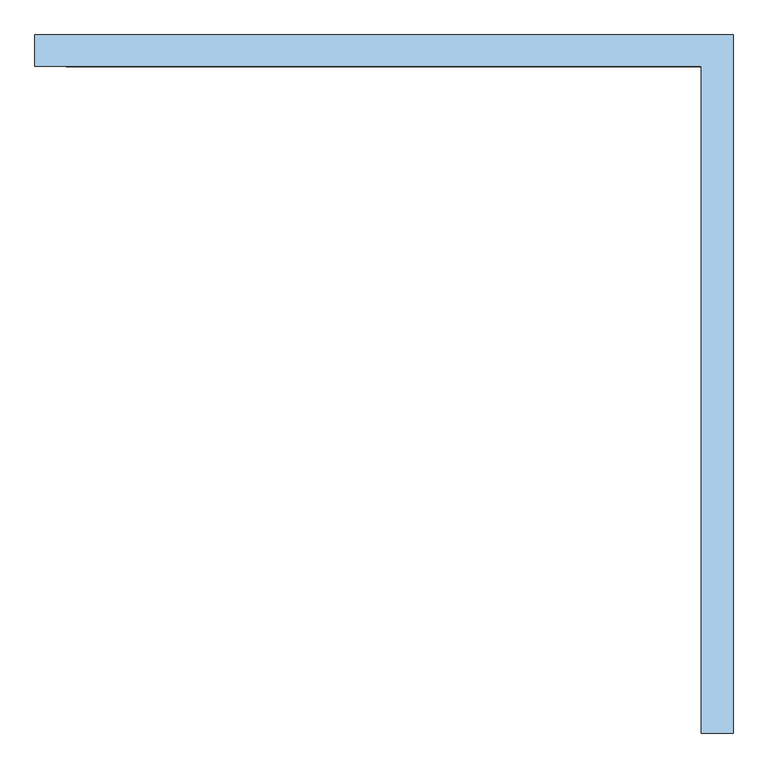
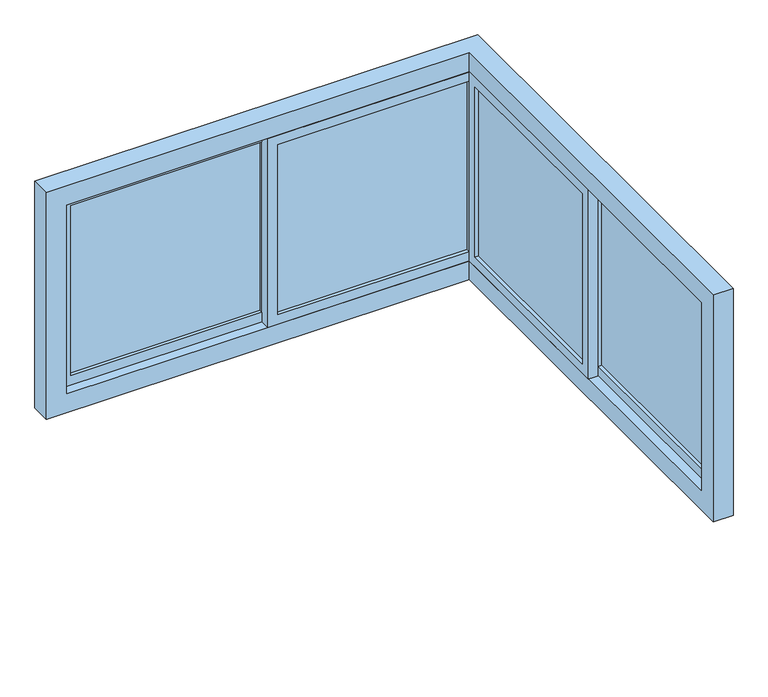
"""IFC4 building model written with IfcOpenShell, lengths in millimetres: window geometry, .CC_ND 300_JANELA DE CANTO_4 FOLHAS DE CORRER_VIDRO : 1.20F X 1.20E X 0.60H."""

from ifc_helpers import new_model, si_unit, frame, origin, place, context, project, spatial, polyline, outline, extrude, faceted_brep, source, transform, mapped, element, save


def window_65d6727e(model_context):
    return source(origin(), model_context, "Body", "SolidModel", [
        extrude(outline(polyline([(-516.0, 1950.0), (-516.0, 1450.0), (-1032.0, 1450.0), (-1032.0, 1950.0), (-516.0, 1950.0)]), holes=[polyline([(-541.0, 1925.0), (-1007.0, 1925.0), (-1007.0, 1475.0), (-541.0, 1475.0), (-541.0, 1925.0)])]), frame((482.0, 0.0, 0.0), z_axis=(1.0, 0.0, 0.0), x_axis=(0.0, 1.0, 0.0)), (0.0, 0.0, 1.0), 25.0),
        extrude(outline(polyline([(490.5, -541.0), (498.5, -541.0), (498.5, -1007.0), (490.5, -1007.0), (490.5, -541.0)])), frame((0.0, 0.0, 1475.0), z_axis=(0.0, 0.0, 1.0), x_axis=(1.0, 0.0, 0.0)), (0.0, 0.0, 1.0), 450.0),
        extrude(outline(polyline([(-25.0, 1950.0), (-25.0, 1450.0), (-541.0, 1450.0), (-541.0, 1950.0), (-25.0, 1950.0)]), holes=[polyline([(-50.0, 1925.0), (-516.0, 1925.0), (-516.0, 1475.0), (-50.0, 1475.0), (-50.0, 1925.0)])]), frame((457.0, 0.0, 0.0), z_axis=(1.0, 0.0, 0.0), x_axis=(0.0, 1.0, 0.0)), (0.0, 0.0, 1.0), 25.0),
        extrude(outline(polyline([(465.5, -50.0), (473.5, -50.0), (473.5, -516.0), (465.5, -516.0), (465.5, -50.0)])), frame((0.0, 0.0, 1475.0), z_axis=(0.0, 0.0, 1.0), x_axis=(1.0, 0.0, 0.0)), (0.0, 0.0, 1.0), 450.0),
        extrude(outline(polyline([(1950.0, 482.0), (1950.0, -46.5), (1450.0, -46.5), (1450.0, 482.0), (1950.0, 482.0)]), holes=[polyline([(1925.0, 457.0), (1475.0, 457.0), (1475.0, -21.5), (1925.0, -21.5), (1925.0, 457.0)])]), frame((0.0, -25.0, 0.0), z_axis=(0.0, 1.0, 0.0), x_axis=(0.0, 0.0, 1.0)), (0.0, 0.0, 1.0), 25.0),
        extrude(outline(polyline([(457.0, -8.5), (457.0, -16.5), (-21.5, -16.5), (-21.5, -8.5), (457.0, -8.5)])), frame((0.0, 0.0, 1475.0), z_axis=(0.0, 0.0, 1.0), x_axis=(1.0, 0.0, 0.0)), (0.0, 0.0, 1.0), 450.0),
        extrude(outline(polyline([(1950.0, -21.5), (1950.0, -550.0), (1450.0, -550.0), (1450.0, -21.5), (1950.0, -21.5)]), holes=[polyline([(1925.0, -46.5), (1475.0, -46.5), (1475.0, -525.0), (1925.0, -525.0), (1925.0, -46.5)])]), frame((0.0, 0.0, 0.0), z_axis=(0.0, 1.0, 0.0), x_axis=(0.0, 0.0, 1.0)), (0.0, 0.0, 1.0), 25.0),
        extrude(outline(polyline([(-46.5, 16.5), (-46.5, 8.5), (-525.0, 8.5), (-525.0, 16.5), (-46.5, 16.5)])), frame((0.0, 0.0, 1475.0), z_axis=(0.0, 0.0, 1.0), x_axis=(1.0, 0.0, 0.0)), (0.0, 0.0, 1.0), 450.0),
        faceted_brep([(457.0, -1082.0, 1400.0), (457.0, -1082.0, 2000.0), (457.0, -25.0, 2000.0), (457.0, -25.0, 1950.0), (457.0, -1032.0, 1950.0), (457.0, -1032.0, 1450.0), (457.0, -25.0, 1450.0), (457.0, -25.0, 1400.0), (507.0, -1082.0, 1400.0), (507.0, -1082.0, 2000.0), (507.0, -1032.0, 1950.0), (507.0, -1032.0, 1450.0), (507.0, 25.0, 1450.0), (-550.0, 25.0, 1450.0), (-550.0, -25.0, 1450.0), (-600.0, -25.0, 2000.0), (-600.0, -25.0, 1400.0), (-550.0, -25.0, 1950.0), (507.0, 25.0, 1400.0), (-600.0, 25.0, 1400.0), (507.0, 25.0, 1950.0), (507.0, 25.0, 2000.0), (-550.0, 25.0, 1950.0), (-600.0, 25.0, 2000.0)], [[[0, 1, 2, 3, 4, 5, 6, 7]], [[1, 0, 8, 9]], [[5, 4, 10, 11]], [[5, 11, 12, 13, 14, 6]], [[15, 16, 7, 6, 14, 17, 3, 2]], [[18, 8, 0, 7, 16, 19]], [[12, 11, 10, 20, 21, 9, 8, 18]], [[21, 20, 22, 13, 12, 18, 19, 23]], [[17, 14, 13, 22]], [[16, 15, 23, 19]], [[20, 10, 4, 3, 17, 22]], [[1, 9, 21, 23, 15, 2]]]),
    ])


if __name__ == "__main__":
    model = new_model("IFC4")
    model_context = context("Model", 3, world=origin())
    ifc_project = project(units=[si_unit("LENGTHUNIT", "METRE", prefix="MILLI")], contexts=[model_context])
    site = spatial("IfcSite", under=ifc_project)
    building = spatial("IfcBuilding", under=site)
    placement = place(None, origin())
    window_shape = window_65d6727e(model_context)
    element("IfcWindow", 1, ObjectType=".CC_ND 300_JANELA DE CANTO_4 FOLHAS DE CORRER_VIDRO : 1.20F X 1.20E X 0.60H", at=placement, inside=building, context=model_context, shape_type="MappedRepresentation", body=[
        mapped(window_shape, transform((0.0, 0.0, 0.0), x_axis=(1.0, 0.0, 0.0), y_axis=(0.0, 1.0, 0.0), z_axis=(0.0, 0.0, 1.0))),
    ])
    save(model, "model.ifc")

# Revit data of these elements
# Type ".CC_ND 300_JANELA DE CANTO_4 FOLHAS DE CORRER_VIDRO : 1.20F X 1.20E X 0.60H"
#   Type Mark = "57"
#   Vidro_Espessura [instance default] = 0.008 m
#   Painéis_Altura [instance default] = 0.50 m
#   Moldura Painéis_Espessura [instance default] = 0.025 m
#   Moldura Janela_Largura [instance default] = 0.05 m
#   Painéis Frente_Largura [instance default] = 0.5375 m
#   Painéis Esquerda_Largura [instance default] = 0.525 m
#   Moldura Janela_Extensão Interior [instance default] = 0.025 m
#   Moldura Janela_Extensão Frente [instance default] = 0.025 m
#   Rough Width = 2.40 m
#   Largura Frontal = 1.20 m
#   Largura Esquerda = 1.20 m
#   Moldura Painéis_Largura [instance default] = 0.025 m
#   Espessura da parede [instance default] = 0.20 m
#   Moldura Janela_Espessura [instance default] = 0.05 m
#   Height = 0.60 m
#   Altura-padrão do peitoril [instance default] = 1.40 m
#   Width = 2.40 m
#   Vidro [instance default] = none
#   Moldura/Painéis [instance default] = none
#   Rough Height = 0
#   Wall Closure = (empty or 0)
# Element 1 (IfcWindow, ".CC_ND 300_JANELA DE CANTO_4 FOLHAS DE CORRER_VIDRO : 1.20F X 1.20E X 0.60H")
#   Painéis Frente_Largura = 0.5285 m
#   Painéis Esquerda_Largura = 0.516 m
#   Espessura da parede = 0.236 m
#   Vidro = .VIDRO GENÉRICO
#   Moldura/Painéis = .ALUMÍNIO COM PINTURA ELETROSTÁTICA BRANCA
#   Materials on its faces: ".ALUMÍNIO COM PINTURA ELETROSTÁTICA BRANCA", ".VIDRO GENÉRICO"
# Materials
#   ".ALUMÍNIO COM PINTURA ELETROSTÁTICA BRANCA": class "CC_METAIS", colour RGB 241 241 241, transparency 0, Cost = 0
#   ".VIDRO GENÉRICO": class ".CC_VIDRO", colour RGB 0 128 192, transparency 0.9, Description = "Vidro comum", Cost = 0
